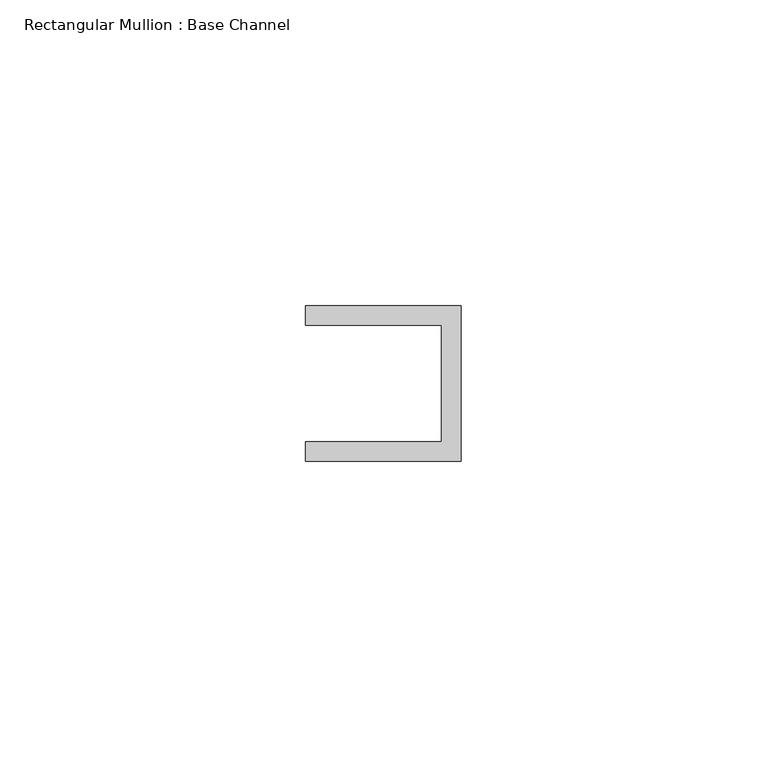
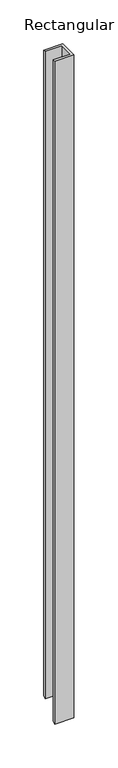
"""IFC4 building model written with IfcOpenShell, lengths in millimetres: member geometry, Rectangular Mullion : Base Channel."""

import ifcopenshell
import ifcopenshell.guid

model = None  # the IFC model being written
_history = None  # IfcOwnerHistory: only IFC2X3 demands one
_inside = {}  # id of a spatial element -> (the spatial element, [elements in it])
_under = {}  # id of a project, library or spatial element -> (it, [spatial elements below it])
_declared = {}  # id of a project -> (the project, [libraries it declares])
_typed = {}  # id of a type object -> (the type object, [elements of that type])
_made_of = {}  # id of a material, layer set ... -> (it, [elements and type objects made of it])


def new_model(schema):
    """Start an empty IFC model of exactly this schema.

    Asked for "IFC4X3", IfcOpenShell would pick the latest addendum, in which some entities
    have other attributes; the version numbers below select the first issue.
    IFC2X3 requires an IfcOwnerHistory on every rooted entity: one is made here for all.
    """
    global model, _history
    if schema == "IFC4X3":
        model = ifcopenshell.file(schema_version=(4, 3, 0, 0))
    else:
        model = ifcopenshell.file(schema=schema)
    _inside.clear()
    _under.clear()
    _declared.clear()
    _typed.clear()
    _made_of.clear()
    _history = None
    if model.schema == "IFC2X3":
        org = make("IfcOrganization", Name="unknown")
        user = make(
            "IfcPersonAndOrganization",
            ThePerson=make("IfcPerson", FamilyName="unknown"),
            TheOrganization=org,
        )
        app = make(
            "IfcApplication",
            ApplicationDeveloper=org,
            Version="unknown",
            ApplicationFullName="unknown",
            ApplicationIdentifier="unknown",
        )
        _history = make(
            "IfcOwnerHistory",
            OwningUser=user,
            OwningApplication=app,
            ChangeAction="ADDED",
            CreationDate=0,
        )
    return model


def make(cls, **values):
    """One entity of the class cls with the attributes given. An attribute that is None is left unset."""
    return model.create_entity(
        cls, **{name: value for name, value in values.items() if value is not None}
    )


def rooted(cls, **values):
    """An entity with a GlobalId (a new one), such as an element, a storey or a relation."""
    return make(cls, GlobalId=ifcopenshell.guid.new(), OwnerHistory=_history, **values)


def si_unit(unit_type, name, prefix=None):
    """IfcSIUnit, for example si_unit("LENGTHUNIT", "METRE", prefix="MILLI")."""
    return make("IfcSIUnit", UnitType=unit_type, Prefix=prefix, Name=name)


def assignment(units):
    """IfcUnitAssignment: the units of a project."""
    return None if units is None else make("IfcUnitAssignment", Units=units)


def point(xyz):
    """IfcCartesianPoint."""
    return None if xyz is None else make("IfcCartesianPoint", Coordinates=xyz)


def direction(xyz):
    """IfcDirection."""
    return None if xyz is None else make("IfcDirection", DirectionRatios=xyz)


def frame(location, z_axis=None, x_axis=None):
    """IfcAxis2Placement3D, a coordinate frame: its origin and axes. An axis left out is left unset."""
    return make(
        "IfcAxis2Placement3D",
        Location=point(location),
        Axis=direction(z_axis),
        RefDirection=direction(x_axis),
    )


def origin():
    """The frame at (0, 0, 0) with its axes left unset."""
    return frame((0.0, 0.0, 0.0))


def place(relative_to, where):
    """IfcLocalPlacement: puts the frame where relative to a parent placement (None: the world)."""
    return make(
        "IfcLocalPlacement", PlacementRelTo=relative_to, RelativePlacement=where
    )


def context(
    kind, dimensions, precision=None, world=None, true_north=None, identifier=None
):
    """IfcGeometricRepresentationContext, for example the 3D "Model" context."""
    return make(
        "IfcGeometricRepresentationContext",
        ContextIdentifier=identifier,
        ContextType=kind,
        CoordinateSpaceDimension=dimensions,
        Precision=precision,
        WorldCoordinateSystem=world,
        TrueNorth=true_north,
    )


def project(units=None, contexts=None):
    """IfcProject with its units and contexts."""
    return rooted(
        "IfcProject",
        Name="project",
        RepresentationContexts=contexts,
        UnitsInContext=assignment(units),
    )


def spatial(cls, under=None, at=None, **own):
    """A site, building, storey or space (cls), placed at a placement, below another one or the project."""
    s = rooted(cls, ObjectPlacement=at, **own)
    if under is not None:
        _under.setdefault(under.id(), (under, []))[1].append(s)
    return s


def faces_of(points, faces, orient=None, outer=None):
    """IfcFace entities. A face is a list of loops; a loop is a list of indices into points, from 0.

    orient and outer hold one flag for each loop. By default every Orientation is true, the
    first loop of a face is its IfcFaceOuterBound and the others are IfcFaceBound.
    """
    made = []
    for i, loops in enumerate(faces):
        bounds = []
        for j, loop in enumerate(loops):
            is_outer = j == 0 if outer is None else outer[i][j]
            bounds.append(
                make(
                    "IfcFaceOuterBound" if is_outer else "IfcFaceBound",
                    Bound=make("IfcPolyLoop", Polygon=[points[k] for k in loop]),
                    Orientation=True if orient is None else orient[i][j],
                )
            )
        made.append(make("IfcFace", Bounds=bounds))
    return made


def faceted_brep(points, faces, orient=None, outer=None, voids=None):
    """IfcFacetedBrep: a solid bounded by flat faces; with voids (closed shells), ...WithVoids."""
    shared = [point(p) for p in points]
    hull = make("IfcClosedShell", CfsFaces=faces_of(shared, faces, orient, outer))
    if voids is None:
        return make("IfcFacetedBrep", Outer=hull)
    return make(
        "IfcFacetedBrepWithVoids",
        Outer=hull,
        Voids=[
            make(cls, CfsFaces=faces_of(shared, fs, o, b)) for cls, fs, o, b in voids
        ],
    )


def shape(context_of_items, identifier, shape_type, items):
    """IfcShapeRepresentation: the items that make up one representation, for example the "Body"."""
    return make(
        "IfcShapeRepresentation",
        ContextOfItems=context_of_items,
        RepresentationIdentifier=identifier,
        RepresentationType=shape_type,
        Items=items,
    )


def source(mapping_origin, context_of_items, identifier, shape_type, items):
    """IfcRepresentationMap: a shape defined once, which mapped items show again and again."""
    return make(
        "IfcRepresentationMap",
        MappingOrigin=mapping_origin,
        MappedRepresentation=shape(context_of_items, identifier, shape_type, items),
    )


def transform(
    local_origin,
    x_axis=None,
    y_axis=None,
    z_axis=None,
    scale=None,
    scale2=None,
    scale3=None,
    uniform=True,
):
    """IfcCartesianTransformationOperator3D, or its non-uniform kind. x_axis, y_axis, z_axis: its Axis1, 2, 3."""
    if uniform:
        return make(
            "IfcCartesianTransformationOperator3D",
            Axis1=direction(x_axis),
            Axis2=direction(y_axis),
            LocalOrigin=point(local_origin),
            Scale=scale,
            Axis3=direction(z_axis),
        )
    return make(
        "IfcCartesianTransformationOperator3DnonUniform",
        Axis1=direction(x_axis),
        Axis2=direction(y_axis),
        LocalOrigin=point(local_origin),
        Scale=scale,
        Axis3=direction(z_axis),
        Scale2=scale2,
        Scale3=scale3,
    )


def mapped(mapping_source, mapping_target):
    """IfcMappedItem: shows the shape of a source again, moved by a transform."""
    return make(
        "IfcMappedItem", MappingSource=mapping_source, MappingTarget=mapping_target
    )


def made_of(thing, what):
    """Note that an element or type object is made of a material, layer set ...; save() writes the relation."""
    if what is not None:
        _made_of.setdefault(what.id(), (what, []))[1].append(thing)
    return thing


def element(
    cls,
    number,
    at=None,
    inside=None,
    cuts=None,
    type_object=None,
    material=None,
    context=None,
    identifier="Body",
    shape_type=None,
    held_by="IfcProductDefinitionShape",
    body=None,
    shapes=None,
    **own,
):
    """One element of the class cls, such as IfcWall. Its Tag is "e" and its number.

    at: its placement. inside: the storey or other place that contains it. cuts: it is an
    opening in that element (IfcRelVoidsElement). A single representation is given by context,
    identifier, shape_type and body (its items); several are given by shapes. held_by: the class
    of the entity that holds the representations. save() writes the other relations.
    """
    e = rooted(cls, Tag="e%d" % number, ObjectPlacement=at, **own)
    if body is not None:
        shapes = [shape(context, identifier, shape_type, body)]
    if shapes is not None:
        e.Representation = make(held_by, Representations=shapes)
    if inside is not None:
        _inside.setdefault(inside.id(), (inside, []))[1].append(e)
    if cuts is not None:
        rooted(
            "IfcRelVoidsElement", RelatingBuildingElement=cuts, RelatedOpeningElement=e
        )
    if type_object is not None:
        _typed.setdefault(type_object.id(), (type_object, []))[1].append(e)
    return made_of(e, material)


def aggregate(whole, parts):
    """IfcRelAggregates: a whole, such as a stair, and the parts it consists of."""
    return rooted("IfcRelAggregates", RelatingObject=whole, RelatedObjects=parts)


def save(model, path):
    """Write the relations noted so far, then the file.

    IfcRelAggregates (storeys below a building ...), IfcRelContainedInSpatialStructure (elements
    in a storey), IfcRelDefinesByType, IfcRelAssociatesMaterial and IfcRelDeclares: one each for
    every whole, place, type object, material and project.
    """
    for whole, parts in _under.values():
        aggregate(whole, parts)
    for where, things in _inside.values():
        rooted(
            "IfcRelContainedInSpatialStructure",
            RelatedElements=things,
            RelatingStructure=where,
        )
    for kind, things in _typed.values():
        rooted("IfcRelDefinesByType", RelatedObjects=things, RelatingType=kind)
    for what, things in _made_of.values():
        rooted("IfcRelAssociatesMaterial", RelatedObjects=things, RelatingMaterial=what)
    for by, libraries in _declared.values():
        rooted("IfcRelDeclares", RelatingContext=by, RelatedDefinitions=libraries)
    model.write(path)


def rectangular_mullion_base_channel_798368e3(model_context):
    return source(origin(), model_context, "Body", "Brep", [
        faceted_brep([(0.0, -12.7, 0.0), (0.0, 12.7, 0.0), (-25.4, 12.7, 0.0), (-25.4, 9.525, 0.0), (-3.175, 9.525, 0.0), (-3.175, -9.525, 0.0), (-25.4, -9.525, 0.0), (-25.4, -12.7, 0.0), (0.0, -12.7, -927.1000003), (0.0, 12.7, -901.7000003), (-25.4, 12.7, -901.7000003), (-25.4, 9.525, -904.8750003), (-3.175, 9.525, -904.8750003), (-3.175, -9.525, -923.9250003), (-25.4, -9.525, -923.9250003), (-25.4, -12.7, -927.1000003)], [[[0, 1, 2, 3, 4, 5, 6, 7]], [[1, 0, 8, 9]], [[2, 1, 9, 10]], [[3, 2, 10, 11]], [[4, 3, 11, 12]], [[5, 4, 12, 13]], [[6, 5, 13, 14]], [[7, 6, 14, 15]], [[0, 7, 15, 8]], [[8, 15, 14, 13, 12, 11, 10, 9]]]),
    ])


if __name__ == "__main__":
    model = new_model("IFC4")
    model_context = context("Model", 3, world=origin())
    ifc_project = project(units=[si_unit("LENGTHUNIT", "METRE", prefix="MILLI")], contexts=[model_context])
    site = spatial("IfcSite", under=ifc_project)
    building = spatial("IfcBuilding", under=site)
    placement = place(None, origin())
    rectangular_mullion_base_channel_shape = rectangular_mullion_base_channel_798368e3(model_context)
    element("IfcMember", 1, ObjectType="Rectangular Mullion : Base Channel", at=placement, inside=building, context=model_context, shape_type="MappedRepresentation", body=[
        mapped(rectangular_mullion_base_channel_shape, transform((0.0, 0.0, 0.0), x_axis=(1.0, 0.0, 0.0), y_axis=(0.0, 1.0, 0.0), z_axis=(0.0, 0.0, 1.0))),
    ])
    save(model, "model.ifc")

# Revit data of these elements
# Type "Rectangular Mullion : Base Channel"
#   built-in parameter 1007322 = 0.0833333 (stored number, unit not read)
#   built-in parameter 1007321 = 0.0416667 (stored number, unit not read)
#   built-in parameter 1007320 = -0.03125 (stored number, unit not read)
# Element 1 (IfcMember, "Rectangular Mullion : Base Channel")
#   Materials on its faces: "ALUM"
# Materials
#   "ALUM": class "Generic", colour RGB 157 157 157, transparency 0, Cost = 0
